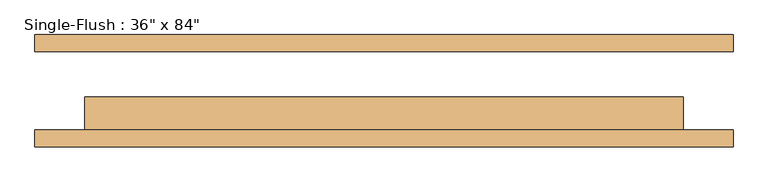
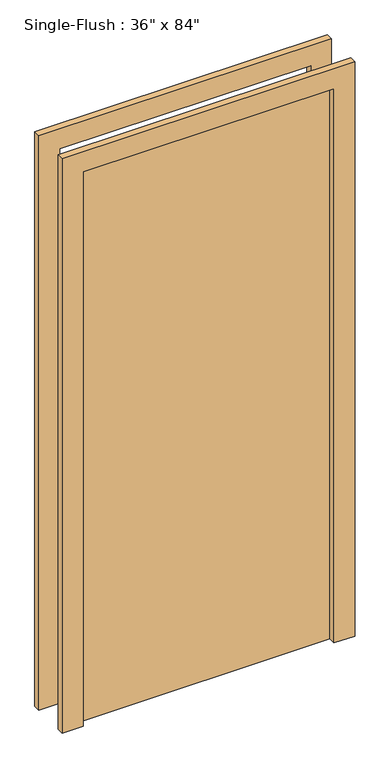
"""IFC4 building model written with IfcOpenShell, lengths in millimetres: door geometry."""

import ifcopenshell
import ifcopenshell.guid

model = None  # the IFC model being written
_history = None  # IfcOwnerHistory: only IFC2X3 demands one
_inside = {}  # id of a spatial element -> (the spatial element, [elements in it])
_under = {}  # id of a project, library or spatial element -> (it, [spatial elements below it])
_declared = {}  # id of a project -> (the project, [libraries it declares])
_typed = {}  # id of a type object -> (the type object, [elements of that type])
_made_of = {}  # id of a material, layer set ... -> (it, [elements and type objects made of it])


def new_model(schema):
    """Start an empty IFC model of exactly this schema.

    Asked for "IFC4X3", IfcOpenShell would pick the latest addendum, in which some entities
    have other attributes; the version numbers below select the first issue.
    IFC2X3 requires an IfcOwnerHistory on every rooted entity: one is made here for all.
    """
    global model, _history
    if schema == "IFC4X3":
        model = ifcopenshell.file(schema_version=(4, 3, 0, 0))
    else:
        model = ifcopenshell.file(schema=schema)
    _inside.clear()
    _under.clear()
    _declared.clear()
    _typed.clear()
    _made_of.clear()
    _history = None
    if model.schema == "IFC2X3":
        org = make("IfcOrganization", Name="unknown")
        user = make(
            "IfcPersonAndOrganization",
            ThePerson=make("IfcPerson", FamilyName="unknown"),
            TheOrganization=org,
        )
        app = make(
            "IfcApplication",
            ApplicationDeveloper=org,
            Version="unknown",
            ApplicationFullName="unknown",
            ApplicationIdentifier="unknown",
        )
        _history = make(
            "IfcOwnerHistory",
            OwningUser=user,
            OwningApplication=app,
            ChangeAction="ADDED",
            CreationDate=0,
        )
    return model


def make(cls, **values):
    """One entity of the class cls with the attributes given. An attribute that is None is left unset."""
    return model.create_entity(
        cls, **{name: value for name, value in values.items() if value is not None}
    )


def rooted(cls, **values):
    """An entity with a GlobalId (a new one), such as an element, a storey or a relation."""
    return make(cls, GlobalId=ifcopenshell.guid.new(), OwnerHistory=_history, **values)


def si_unit(unit_type, name, prefix=None):
    """IfcSIUnit, for example si_unit("LENGTHUNIT", "METRE", prefix="MILLI")."""
    return make("IfcSIUnit", UnitType=unit_type, Prefix=prefix, Name=name)


def assignment(units):
    """IfcUnitAssignment: the units of a project."""
    return None if units is None else make("IfcUnitAssignment", Units=units)


def point(xyz):
    """IfcCartesianPoint."""
    return None if xyz is None else make("IfcCartesianPoint", Coordinates=xyz)


def direction(xyz):
    """IfcDirection."""
    return None if xyz is None else make("IfcDirection", DirectionRatios=xyz)


def frame(location, z_axis=None, x_axis=None):
    """IfcAxis2Placement3D, a coordinate frame: its origin and axes. An axis left out is left unset."""
    return make(
        "IfcAxis2Placement3D",
        Location=point(location),
        Axis=direction(z_axis),
        RefDirection=direction(x_axis),
    )


def origin():
    """The frame at (0, 0, 0) with its axes left unset."""
    return frame((0.0, 0.0, 0.0))


def origin_with_axes():
    """The frame at (0, 0, 0) with the z axis (0, 0, 1) and the x axis (1, 0, 0) written out."""
    return frame((0.0, 0.0, 0.0), z_axis=(0.0, 0.0, 1.0), x_axis=(1.0, 0.0, 0.0))


def place(relative_to, where):
    """IfcLocalPlacement: puts the frame where relative to a parent placement (None: the world)."""
    return make(
        "IfcLocalPlacement", PlacementRelTo=relative_to, RelativePlacement=where
    )


def context(
    kind, dimensions, precision=None, world=None, true_north=None, identifier=None
):
    """IfcGeometricRepresentationContext, for example the 3D "Model" context."""
    return make(
        "IfcGeometricRepresentationContext",
        ContextIdentifier=identifier,
        ContextType=kind,
        CoordinateSpaceDimension=dimensions,
        Precision=precision,
        WorldCoordinateSystem=world,
        TrueNorth=true_north,
    )


def project(units=None, contexts=None):
    """IfcProject with its units and contexts."""
    return rooted(
        "IfcProject",
        Name="project",
        RepresentationContexts=contexts,
        UnitsInContext=assignment(units),
    )


def spatial(cls, under=None, at=None, **own):
    """A site, building, storey or space (cls), placed at a placement, below another one or the project."""
    s = rooted(cls, ObjectPlacement=at, **own)
    if under is not None:
        _under.setdefault(under.id(), (under, []))[1].append(s)
    return s


def polyline(points):
    """IfcPolyline through the points."""
    return make("IfcPolyline", Points=[point(p) for p in points])


def outline(outer, holes=None, kind="AREA"):
    """IfcArbitraryClosedProfileDef: a profile drawn as a closed curve; with holes, ...WithVoids."""
    if holes is None:
        return make("IfcArbitraryClosedProfileDef", ProfileType=kind, OuterCurve=outer)
    return make(
        "IfcArbitraryProfileDefWithVoids",
        ProfileType=kind,
        OuterCurve=outer,
        InnerCurves=holes,
    )


def extrude(swept, where, along, depth):
    """IfcExtrudedAreaSolid: the profile swept, set in the frame where, extruded along a direction by depth."""
    return make(
        "IfcExtrudedAreaSolid",
        SweptArea=swept,
        Position=where,
        ExtrudedDirection=direction(along),
        Depth=depth,
    )


def shape(context_of_items, identifier, shape_type, items):
    """IfcShapeRepresentation: the items that make up one representation, for example the "Body"."""
    return make(
        "IfcShapeRepresentation",
        ContextOfItems=context_of_items,
        RepresentationIdentifier=identifier,
        RepresentationType=shape_type,
        Items=items,
    )


def source(mapping_origin, context_of_items, identifier, shape_type, items):
    """IfcRepresentationMap: a shape defined once, which mapped items show again and again."""
    return make(
        "IfcRepresentationMap",
        MappingOrigin=mapping_origin,
        MappedRepresentation=shape(context_of_items, identifier, shape_type, items),
    )


def transform(
    local_origin,
    x_axis=None,
    y_axis=None,
    z_axis=None,
    scale=None,
    scale2=None,
    scale3=None,
    uniform=True,
):
    """IfcCartesianTransformationOperator3D, or its non-uniform kind. x_axis, y_axis, z_axis: its Axis1, 2, 3."""
    if uniform:
        return make(
            "IfcCartesianTransformationOperator3D",
            Axis1=direction(x_axis),
            Axis2=direction(y_axis),
            LocalOrigin=point(local_origin),
            Scale=scale,
            Axis3=direction(z_axis),
        )
    return make(
        "IfcCartesianTransformationOperator3DnonUniform",
        Axis1=direction(x_axis),
        Axis2=direction(y_axis),
        LocalOrigin=point(local_origin),
        Scale=scale,
        Axis3=direction(z_axis),
        Scale2=scale2,
        Scale3=scale3,
    )


def mapped(mapping_source, mapping_target):
    """IfcMappedItem: shows the shape of a source again, moved by a transform."""
    return make(
        "IfcMappedItem", MappingSource=mapping_source, MappingTarget=mapping_target
    )


def made_of(thing, what):
    """Note that an element or type object is made of a material, layer set ...; save() writes the relation."""
    if what is not None:
        _made_of.setdefault(what.id(), (what, []))[1].append(thing)
    return thing


def element(
    cls,
    number,
    at=None,
    inside=None,
    cuts=None,
    type_object=None,
    material=None,
    context=None,
    identifier="Body",
    shape_type=None,
    held_by="IfcProductDefinitionShape",
    body=None,
    shapes=None,
    **own,
):
    """One element of the class cls, such as IfcWall. Its Tag is "e" and its number.

    at: its placement. inside: the storey or other place that contains it. cuts: it is an
    opening in that element (IfcRelVoidsElement). A single representation is given by context,
    identifier, shape_type and body (its items); several are given by shapes. held_by: the class
    of the entity that holds the representations. save() writes the other relations.
    """
    e = rooted(cls, Tag="e%d" % number, ObjectPlacement=at, **own)
    if body is not None:
        shapes = [shape(context, identifier, shape_type, body)]
    if shapes is not None:
        e.Representation = make(held_by, Representations=shapes)
    if inside is not None:
        _inside.setdefault(inside.id(), (inside, []))[1].append(e)
    if cuts is not None:
        rooted(
            "IfcRelVoidsElement", RelatingBuildingElement=cuts, RelatedOpeningElement=e
        )
    if type_object is not None:
        _typed.setdefault(type_object.id(), (type_object, []))[1].append(e)
    return made_of(e, material)


def aggregate(whole, parts):
    """IfcRelAggregates: a whole, such as a stair, and the parts it consists of."""
    return rooted("IfcRelAggregates", RelatingObject=whole, RelatedObjects=parts)


def save(model, path):
    """Write the relations noted so far, then the file.

    IfcRelAggregates (storeys below a building ...), IfcRelContainedInSpatialStructure (elements
    in a storey), IfcRelDefinesByType, IfcRelAssociatesMaterial and IfcRelDeclares: one each for
    every whole, place, type object, material and project.
    """
    for whole, parts in _under.values():
        aggregate(whole, parts)
    for where, things in _inside.values():
        rooted(
            "IfcRelContainedInSpatialStructure",
            RelatedElements=things,
            RelatingStructure=where,
        )
    for kind, things in _typed.values():
        rooted("IfcRelDefinesByType", RelatedObjects=things, RelatingType=kind)
    for what, things in _made_of.values():
        rooted("IfcRelAssociatesMaterial", RelatedObjects=things, RelatingMaterial=what)
    for by, libraries in _declared.values():
        rooted("IfcRelDeclares", RelatingContext=by, RelatedDefinitions=libraries)
    model.write(path)


def door_805e9a83(model_context):
    return source(origin(), model_context, "Body", "SweptSolid", [
        extrude(outline(polyline([(2209.8, -533.4), (0.0, -533.4), (0.0, -457.2), (2133.6, -457.2), (2133.6, 457.2), (0.0, 457.2), (0.0, 533.4), (2209.8, 533.4), (2209.8, -533.4)])), frame((0.0, -85.725, 0.0), z_axis=(0.0, 1.0, 0.0), x_axis=(0.0, 0.0, 1.0)), (0.0, 0.0, 1.0), 25.4),
        extrude(outline(polyline([(2209.8, 533.4), (2209.8, -533.4), (0.0, -533.4), (0.0, -457.2), (2133.6, -457.2), (2133.6, 457.2), (0.0, 457.2), (0.0, 533.4), (2209.8, 533.4)])), frame((0.0, 60.325, 0.0), z_axis=(0.0, 1.0, 0.0), x_axis=(0.0, 0.0, 1.0)), (0.0, 0.0, 1.0), 25.4),
        extrude(outline(polyline([(457.2, -9.525), (457.2, -60.325), (-457.2, -60.325), (-457.2, -9.525), (457.2, -9.525)])), origin_with_axes(), (0.0, 0.0, 1.0), 2133.6),
    ])


if __name__ == "__main__":
    model = new_model("IFC4")
    model_context = context("Model", 3, world=origin())
    ifc_project = project(units=[si_unit("LENGTHUNIT", "METRE", prefix="MILLI")], contexts=[model_context])
    site = spatial("IfcSite", under=ifc_project)
    building = spatial("IfcBuilding", under=site)
    placement = place(None, origin())
    door_shape = door_805e9a83(model_context)
    element("IfcDoor", 1, ObjectType="Single-Flush : 36\" x 84\"", at=placement, inside=building, context=model_context, shape_type="MappedRepresentation", body=[
        mapped(door_shape, transform((0.0, 0.0, 0.0), x_axis=(1.0, 0.0, 0.0), y_axis=(0.0, 1.0, 0.0), z_axis=(0.0, 0.0, 1.0))),
    ])
    save(model, "model.ifc")

# Revit data of these elements
# Type "Single-Flush : 36\" x 84\""
#   Type Mark = "1"
#   Assembly Code = "C1020"
#   Thickness = 0' - 2"
#   Height = 7' - 0"
#   Trim Projection Ext = 0' - 1"
#   Trim Projection Int = 0' - 1"
#   Trim Width = 0' - 3"
#   Width = 3' - 0"
#   Door Material = none
#   Frame Material = none
#   Function = (empty or 0)
#   Wall Closure = (empty or 0)
